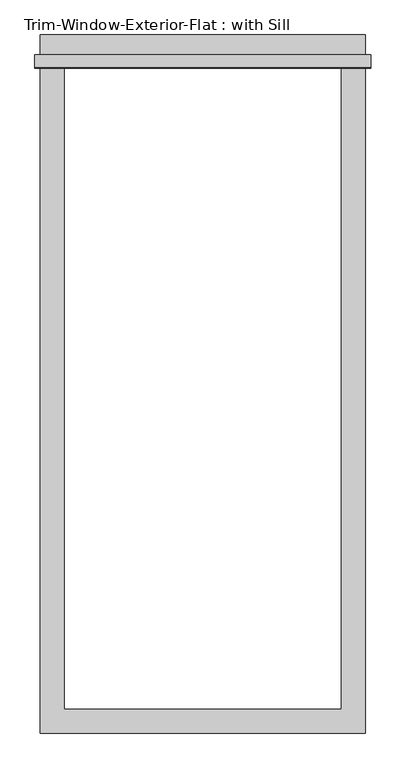
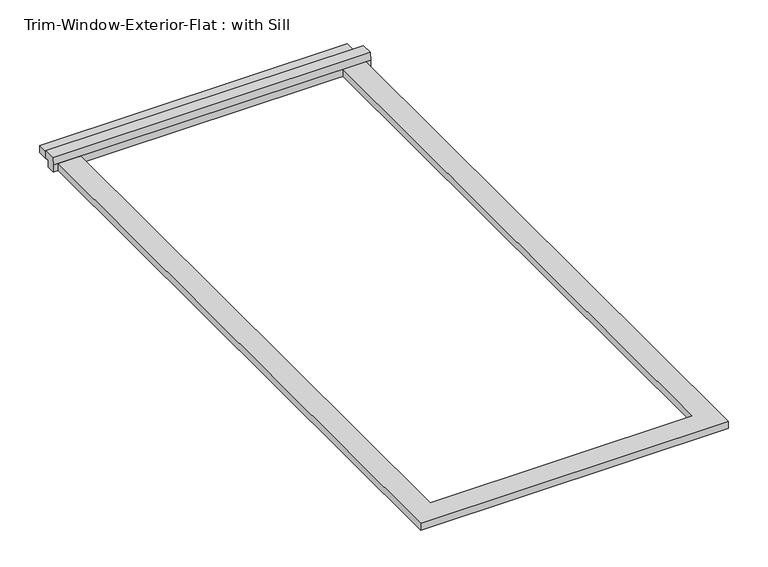
"""IFC4 building model written with IfcOpenShell, lengths in millimetres: proxy geometry, Trim-Window-Exterior-Flat : with Sill."""

from ifc_helpers import new_model, si_unit, frame, origin, origin_with_axes, place, context, project, spatial, polyline, outline, extrude, source, transform, mapped, element, save


def trim_window_exterior_flat_with_sill_732fd250(model_context):
    return source(origin(), model_context, "Body", "SweptSolid", [
        extrude(outline(polyline([(387.35, 1546.1823709), (-387.35, 1546.1823709), (-387.35, 1603.3323709), (387.35, 1603.3323709), (387.35, 1546.1823709)])), origin_with_axes(), (0.0, 0.0, 1.0), 19.05),
        extrude(outline(polyline([(1555.75, 38.1), (1555.75, 19.05), (1546.1823709, 19.05), (1546.1823709, 0.0), (1524.0, 0.0), (1524.0, 19.05), (1526.4580645, 38.1), (1555.75, 38.1)])), frame((-400.05, 0.0, 0.0), z_axis=(1.0, 0.0, 0.0), x_axis=(0.0, 1.0, 0.0)), (0.0, 0.0, 1.0), 800.1),
        extrude(outline(polyline([(-387.35, -57.15), (-387.35, 1524.0), (-330.2, 1524.0), (-330.2, 0.0), (330.2, 0.0), (330.2, 1524.0), (387.35, 1524.0), (387.35, -57.15), (-387.35, -57.15)])), origin_with_axes(), (0.0, 0.0, 1.0), 19.05),
    ])


if __name__ == "__main__":
    model = new_model("IFC4")
    model_context = context("Model", 3, world=origin())
    ifc_project = project(units=[si_unit("LENGTHUNIT", "METRE", prefix="MILLI")], contexts=[model_context])
    site = spatial("IfcSite", under=ifc_project)
    building = spatial("IfcBuilding", under=site)
    placement = place(None, origin())
    trim_window_exterior_flat_with_sill_shape = trim_window_exterior_flat_with_sill_732fd250(model_context)
    element("IfcBuildingElementProxy", 1, Name="Trim-Window-Exterior-Flat : with Sill", ObjectType="Trim-Window-Exterior-Flat : with Sill", at=placement, inside=building, context=model_context, shape_type="MappedRepresentation", body=[
        mapped(trim_window_exterior_flat_with_sill_shape, transform((0.0, 0.0, 0.0), x_axis=(1.0, 0.0, 0.0), y_axis=(0.0, 1.0, 0.0), z_axis=(0.0, 0.0, 1.0))),
    ])
    save(model, "model.ifc")

# Revit data of these elements
# Type "Trim-Window-Exterior-Flat : with Sill"
#   Trim Width = 0' - 2 1/4"
#   Trim Thickness_Picture Frame = 0' - 1 1/4"
#   Trim Thickness_with Sill = 0' - 0 3/4"
#   Sill Thickness = 0' - 1 1/4"
#   Opening Width [instance default] = 2' - 0"
#   Opening Height [instance default] = 3' - 0"
#   Default Elevation = 4' - 0"
#   Sill = yes
#   Picture Frame = no
#   Trim Material [instance default] = none
# Element 1 (IfcBuildingElementProxy, "Trim-Window-Exterior-Flat : with Sill")
#   Opening Width = 2' - 2"
#   Opening Height = 5' - 0"
#   Trim Material = Clad - White
#   Materials on its faces: "Clad - White"
# Materials
#   "Clad - White": class "Wood", colour RGB 242 242 238, transparency 0, Cost = 0
